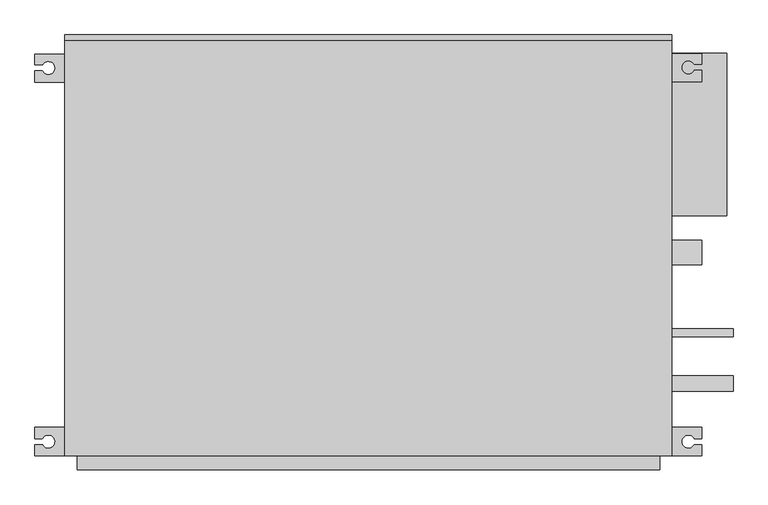
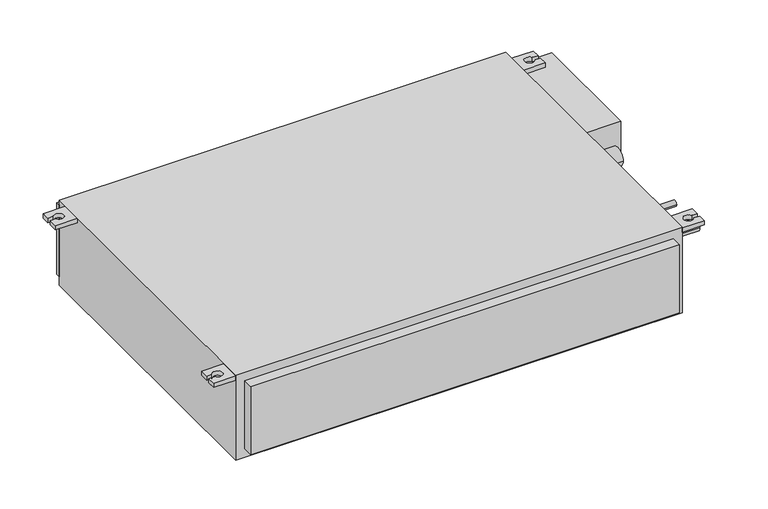
"""IFC4 building model written with IfcOpenShell, lengths in millimetres: proxy geometry, PEFY-P-NMSU-E_Low_Profile_Ducted : PEFY-P15NMSU-E."""

import ifcopenshell
import ifcopenshell.guid

model = None  # the IFC model being written
_history = None  # IfcOwnerHistory: only IFC2X3 demands one
_inside = {}  # id of a spatial element -> (the spatial element, [elements in it])
_under = {}  # id of a project, library or spatial element -> (it, [spatial elements below it])
_declared = {}  # id of a project -> (the project, [libraries it declares])
_typed = {}  # id of a type object -> (the type object, [elements of that type])
_made_of = {}  # id of a material, layer set ... -> (it, [elements and type objects made of it])


def new_model(schema):
    """Start an empty IFC model of exactly this schema.

    Asked for "IFC4X3", IfcOpenShell would pick the latest addendum, in which some entities
    have other attributes; the version numbers below select the first issue.
    IFC2X3 requires an IfcOwnerHistory on every rooted entity: one is made here for all.
    """
    global model, _history
    if schema == "IFC4X3":
        model = ifcopenshell.file(schema_version=(4, 3, 0, 0))
    else:
        model = ifcopenshell.file(schema=schema)
    _inside.clear()
    _under.clear()
    _declared.clear()
    _typed.clear()
    _made_of.clear()
    _history = None
    if model.schema == "IFC2X3":
        org = make("IfcOrganization", Name="unknown")
        user = make(
            "IfcPersonAndOrganization",
            ThePerson=make("IfcPerson", FamilyName="unknown"),
            TheOrganization=org,
        )
        app = make(
            "IfcApplication",
            ApplicationDeveloper=org,
            Version="unknown",
            ApplicationFullName="unknown",
            ApplicationIdentifier="unknown",
        )
        _history = make(
            "IfcOwnerHistory",
            OwningUser=user,
            OwningApplication=app,
            ChangeAction="ADDED",
            CreationDate=0,
        )
    return model


def make(cls, **values):
    """One entity of the class cls with the attributes given. An attribute that is None is left unset."""
    return model.create_entity(
        cls, **{name: value for name, value in values.items() if value is not None}
    )


def rooted(cls, **values):
    """An entity with a GlobalId (a new one), such as an element, a storey or a relation."""
    return make(cls, GlobalId=ifcopenshell.guid.new(), OwnerHistory=_history, **values)


def si_unit(unit_type, name, prefix=None):
    """IfcSIUnit, for example si_unit("LENGTHUNIT", "METRE", prefix="MILLI")."""
    return make("IfcSIUnit", UnitType=unit_type, Prefix=prefix, Name=name)


def assignment(units):
    """IfcUnitAssignment: the units of a project."""
    return None if units is None else make("IfcUnitAssignment", Units=units)


def point(xyz):
    """IfcCartesianPoint."""
    return None if xyz is None else make("IfcCartesianPoint", Coordinates=xyz)


def direction(xyz):
    """IfcDirection."""
    return None if xyz is None else make("IfcDirection", DirectionRatios=xyz)


def frame(location, z_axis=None, x_axis=None):
    """IfcAxis2Placement3D, a coordinate frame: its origin and axes. An axis left out is left unset."""
    return make(
        "IfcAxis2Placement3D",
        Location=point(location),
        Axis=direction(z_axis),
        RefDirection=direction(x_axis),
    )


def frame_2d(location, x_axis=None):
    """IfcAxis2Placement2D, a coordinate frame in the plane: its origin and x axis."""
    return make(
        "IfcAxis2Placement2D", Location=point(location), RefDirection=direction(x_axis)
    )


def origin():
    """The frame at (0, 0, 0) with its axes left unset."""
    return frame((0.0, 0.0, 0.0))


def origin_with_axes():
    """The frame at (0, 0, 0) with the z axis (0, 0, 1) and the x axis (1, 0, 0) written out."""
    return frame((0.0, 0.0, 0.0), z_axis=(0.0, 0.0, 1.0), x_axis=(1.0, 0.0, 0.0))


def place(relative_to, where):
    """IfcLocalPlacement: puts the frame where relative to a parent placement (None: the world)."""
    return make(
        "IfcLocalPlacement", PlacementRelTo=relative_to, RelativePlacement=where
    )


def context(
    kind, dimensions, precision=None, world=None, true_north=None, identifier=None
):
    """IfcGeometricRepresentationContext, for example the 3D "Model" context."""
    return make(
        "IfcGeometricRepresentationContext",
        ContextIdentifier=identifier,
        ContextType=kind,
        CoordinateSpaceDimension=dimensions,
        Precision=precision,
        WorldCoordinateSystem=world,
        TrueNorth=true_north,
    )


def project(units=None, contexts=None):
    """IfcProject with its units and contexts."""
    return rooted(
        "IfcProject",
        Name="project",
        RepresentationContexts=contexts,
        UnitsInContext=assignment(units),
    )


def spatial(cls, under=None, at=None, **own):
    """A site, building, storey or space (cls), placed at a placement, below another one or the project."""
    s = rooted(cls, ObjectPlacement=at, **own)
    if under is not None:
        _under.setdefault(under.id(), (under, []))[1].append(s)
    return s


def polyline(points):
    """IfcPolyline through the points."""
    return make("IfcPolyline", Points=[point(p) for p in points])


def circle_curve(where, radius):
    """IfcCircle in the frame where."""
    return make("IfcCircle", Position=where, Radius=radius)


def trimmed(basis, trim1, trim2, sense, master):
    """IfcTrimmedCurve: the piece of a basis curve between two trims."""
    return make(
        "IfcTrimmedCurve",
        BasisCurve=basis,
        Trim1=trim1,
        Trim2=trim2,
        SenseAgreement=sense,
        MasterRepresentation=master,
    )


def segment(curve, same_sense, transition):
    """IfcCompositeCurveSegment."""
    return make(
        "IfcCompositeCurveSegment",
        Transition=transition,
        SameSense=same_sense,
        ParentCurve=curve,
    )


def composite_curve(segments, self_intersect=None):
    """IfcCompositeCurve: segments joined end to end."""
    return make("IfcCompositeCurve", Segments=segments, SelfIntersect=self_intersect)


def outline(outer, holes=None, kind="AREA"):
    """IfcArbitraryClosedProfileDef: a profile drawn as a closed curve; with holes, ...WithVoids."""
    if holes is None:
        return make("IfcArbitraryClosedProfileDef", ProfileType=kind, OuterCurve=outer)
    return make(
        "IfcArbitraryProfileDefWithVoids",
        ProfileType=kind,
        OuterCurve=outer,
        InnerCurves=holes,
    )


def extrude(swept, where, along, depth):
    """IfcExtrudedAreaSolid: the profile swept, set in the frame where, extruded along a direction by depth."""
    return make(
        "IfcExtrudedAreaSolid",
        SweptArea=swept,
        Position=where,
        ExtrudedDirection=direction(along),
        Depth=depth,
    )


def shape(context_of_items, identifier, shape_type, items):
    """IfcShapeRepresentation: the items that make up one representation, for example the "Body"."""
    return make(
        "IfcShapeRepresentation",
        ContextOfItems=context_of_items,
        RepresentationIdentifier=identifier,
        RepresentationType=shape_type,
        Items=items,
    )


def source(mapping_origin, context_of_items, identifier, shape_type, items):
    """IfcRepresentationMap: a shape defined once, which mapped items show again and again."""
    return make(
        "IfcRepresentationMap",
        MappingOrigin=mapping_origin,
        MappedRepresentation=shape(context_of_items, identifier, shape_type, items),
    )


def transform(
    local_origin,
    x_axis=None,
    y_axis=None,
    z_axis=None,
    scale=None,
    scale2=None,
    scale3=None,
    uniform=True,
):
    """IfcCartesianTransformationOperator3D, or its non-uniform kind. x_axis, y_axis, z_axis: its Axis1, 2, 3."""
    if uniform:
        return make(
            "IfcCartesianTransformationOperator3D",
            Axis1=direction(x_axis),
            Axis2=direction(y_axis),
            LocalOrigin=point(local_origin),
            Scale=scale,
            Axis3=direction(z_axis),
        )
    return make(
        "IfcCartesianTransformationOperator3DnonUniform",
        Axis1=direction(x_axis),
        Axis2=direction(y_axis),
        LocalOrigin=point(local_origin),
        Scale=scale,
        Axis3=direction(z_axis),
        Scale2=scale2,
        Scale3=scale3,
    )


def mapped(mapping_source, mapping_target):
    """IfcMappedItem: shows the shape of a source again, moved by a transform."""
    return make(
        "IfcMappedItem", MappingSource=mapping_source, MappingTarget=mapping_target
    )


def made_of(thing, what):
    """Note that an element or type object is made of a material, layer set ...; save() writes the relation."""
    if what is not None:
        _made_of.setdefault(what.id(), (what, []))[1].append(thing)
    return thing


def element(
    cls,
    number,
    at=None,
    inside=None,
    cuts=None,
    type_object=None,
    material=None,
    context=None,
    identifier="Body",
    shape_type=None,
    held_by="IfcProductDefinitionShape",
    body=None,
    shapes=None,
    **own,
):
    """One element of the class cls, such as IfcWall. Its Tag is "e" and its number.

    at: its placement. inside: the storey or other place that contains it. cuts: it is an
    opening in that element (IfcRelVoidsElement). A single representation is given by context,
    identifier, shape_type and body (its items); several are given by shapes. held_by: the class
    of the entity that holds the representations. save() writes the other relations.
    """
    e = rooted(cls, Tag="e%d" % number, ObjectPlacement=at, **own)
    if body is not None:
        shapes = [shape(context, identifier, shape_type, body)]
    if shapes is not None:
        e.Representation = make(held_by, Representations=shapes)
    if inside is not None:
        _inside.setdefault(inside.id(), (inside, []))[1].append(e)
    if cuts is not None:
        rooted(
            "IfcRelVoidsElement", RelatingBuildingElement=cuts, RelatedOpeningElement=e
        )
    if type_object is not None:
        _typed.setdefault(type_object.id(), (type_object, []))[1].append(e)
    return made_of(e, material)


def aggregate(whole, parts):
    """IfcRelAggregates: a whole, such as a stair, and the parts it consists of."""
    return rooted("IfcRelAggregates", RelatingObject=whole, RelatedObjects=parts)


def save(model, path):
    """Write the relations noted so far, then the file.

    IfcRelAggregates (storeys below a building ...), IfcRelContainedInSpatialStructure (elements
    in a storey), IfcRelDefinesByType, IfcRelAssociatesMaterial and IfcRelDeclares: one each for
    every whole, place, type object, material and project.
    """
    for whole, parts in _under.values():
        aggregate(whole, parts)
    for where, things in _inside.values():
        rooted(
            "IfcRelContainedInSpatialStructure",
            RelatedElements=things,
            RelatingStructure=where,
        )
    for kind, things in _typed.values():
        rooted("IfcRelDefinesByType", RelatedObjects=things, RelatingType=kind)
    for what, things in _made_of.values():
        rooted("IfcRelAssociatesMaterial", RelatedObjects=things, RelatingMaterial=what)
    for by, libraries in _declared.values():
        rooted("IfcRelDeclares", RelatingContext=by, RelatedDefinitions=libraries)
    model.write(path)


def mechanical_equipment_be926906(model_context):
    return source(origin(), model_context, "Body", "SweptSolid", [
        extrude(outline(composite_curve([segment(polyline([(-544.3, 282.0), (-544.3, 300.9759165), (-532.1454311, 300.9759165)]), True, "CONTINUOUS"), segment(trimmed(circle_curve(frame_2d((-522.2863556, 305.4254582)), 10.8166442), [point((-532.1454311, 300.9759165))], [point((-531.8387803, 310.5))], True, "CARTESIAN"), True, "CONTINUOUS"), segment(polyline([(-531.8387803, 310.5), (-544.3, 310.5), (-544.3, 328.0), (-495.3, 328.0), (-495.3, 282.0), (-544.3, 282.0)]), True, "CONTINUOUS")], self_intersect=False)), frame((0.0, 0.0, 188.55), z_axis=(0.0, 0.0, 1.0), x_axis=(1.0, 0.0, 0.0)), (0.0, 0.0, 1.0), 10.0),
        extrude(outline(composite_curve([segment(polyline([(-544.3, -281.0), (-495.3, -281.0), (-495.3, -327.0), (-544.3, -327.0), (-544.3, -309.5), (-531.8387803, -309.5)]), True, "CONTINUOUS"), segment(trimmed(circle_curve(frame_2d((-522.2863556, -304.4254582)), 10.8166442), [point((-531.8387803, -309.5))], [point((-532.1454311, -299.9759165))], True, "CARTESIAN"), True, "CONTINUOUS"), segment(polyline([(-532.1454311, -299.9759165), (-544.3, -299.9759165), (-544.3, -281.0)]), True, "CONTINUOUS")], self_intersect=False)), frame((0.0, 0.0, 188.55), z_axis=(0.0, 0.0, 1.0), x_axis=(1.0, 0.0, 0.0)), (0.0, 0.0, 1.0), 10.0),
        extrude(outline(composite_curve([segment(polyline([(544.3, 282.9429009), (495.3, 282.9429009), (495.3, 328.9429009), (544.3, 328.9429009), (544.3, 311.4429009), (531.8387803, 311.4429009)]), True, "CONTINUOUS"), segment(trimmed(circle_curve(frame_2d((522.2863556, 306.3683591)), 10.8166442), [point((531.8387803, 311.4429009))], [point((532.1454311, 301.9188174))], True, "CARTESIAN"), True, "CONTINUOUS"), segment(polyline([(532.1454311, 301.9188174), (544.3, 301.9188174), (544.3, 282.9429009)]), True, "CONTINUOUS")], self_intersect=False)), frame((0.0, 0.0, 188.55), z_axis=(0.0, 0.0, 1.0), x_axis=(1.0, 0.0, 0.0)), (0.0, 0.0, 1.0), 10.0),
        extrude(outline(composite_curve([segment(polyline([(544.3, -281.0), (544.3, -299.9759165), (532.1454311, -299.9759165)]), True, "CONTINUOUS"), segment(trimmed(circle_curve(frame_2d((522.2863556, -304.4254582)), 10.8166442), [point((532.1454311, -299.9759165))], [point((531.8387803, -309.5))], True, "CARTESIAN"), True, "CONTINUOUS"), segment(polyline([(531.8387803, -309.5), (544.3, -309.5), (544.3, -327.0), (495.3, -327.0), (495.3, -281.0), (544.3, -281.0)]), True, "CONTINUOUS")], self_intersect=False)), frame((0.0, 0.0, 188.55), z_axis=(0.0, 0.0, 1.0), x_axis=(1.0, 0.0, 0.0)), (0.0, 0.0, 1.0), 10.0),
        extrude(outline(polyline([(495.3, 350.04375), (-495.3, 350.04375), (-495.3, 359.5477547), (495.3, 359.5477547), (495.3, 350.04375)])), frame((0.0, 0.0, 20.0), z_axis=(0.0, 0.0, 1.0), x_axis=(1.0, 0.0, 0.0)), (0.0, 0.0, 1.0), 168.55),
        extrude(outline(composite_curve([segment(trimmed(circle_curve(frame_2d((4.0570991, 59.8)), 20.0421875), [point((-15.9850884, 59.8))], [point((24.0992866, 59.8))], False, "CARTESIAN"), True, "CONTINUOUS"), segment(trimmed(circle_curve(frame_2d((4.0570991, 59.8)), 20.0421875), [point((24.0992866, 59.8))], [point((-15.9850884, 59.8))], False, "CARTESIAN"), True, "CONTINUOUS")], self_intersect=False)), frame((495.3, 0.0, 0.0), z_axis=(1.0, 0.0, 0.0), x_axis=(0.0, 1.0, 0.0)), (0.0, 0.0, 1.0), 26.9863556),
        extrude(outline(composite_curve([segment(trimmed(circle_curve(frame_2d((4.0570991, 149.6)), 20.0421875), [point((-15.9850884, 149.6))], [point((24.0992866, 149.6))], False, "CARTESIAN"), True, "CONTINUOUS"), segment(trimmed(circle_curve(frame_2d((4.0570991, 149.6)), 20.0421875), [point((24.0992866, 149.6))], [point((-15.9850884, 149.6))], False, "CARTESIAN"), True, "CONTINUOUS")], self_intersect=False)), frame((495.3, 0.0, 0.0), z_axis=(1.0, 0.0, 0.0), x_axis=(0.0, 1.0, 0.0)), (0.0, 0.0, 1.0), 49.0),
        extrude(outline(composite_curve([segment(trimmed(circle_curve(frame_2d((-126.5596979, 100.0)), 6.4492188), [point((-133.0089166, 100.0))], [point((-120.1104791, 100.0))], False, "CARTESIAN"), True, "CONTINUOUS"), segment(trimmed(circle_curve(frame_2d((-126.5596979, 100.0)), 6.4492188), [point((-120.1104791, 100.0))], [point((-133.0089166, 100.0))], False, "CARTESIAN"), True, "CONTINUOUS")], self_intersect=False)), frame((495.3, 0.0, 0.0), z_axis=(1.0, 0.0, 0.0), x_axis=(0.0, 1.0, 0.0)), (0.0, 0.0, 1.0), 100.0),
        extrude(outline(composite_curve([segment(trimmed(circle_curve(frame_2d((-209.7540575, 100.0)), 12.7), [point((-222.4540575, 100.0))], [point((-197.0540575, 100.0))], False, "CARTESIAN"), True, "CONTINUOUS"), segment(trimmed(circle_curve(frame_2d((-209.7540575, 100.0)), 12.7), [point((-197.0540575, 100.0))], [point((-222.4540575, 100.0))], False, "CARTESIAN"), True, "CONTINUOUS")], self_intersect=False)), frame((495.3, 0.0, 0.0), z_axis=(1.0, 0.0, 0.0), x_axis=(0.0, 1.0, 0.0)), (0.0, 0.0, 1.0), 100.0),
        extrude(outline(polyline([(585.3, 330.0), (585.3, 64.0570991), (495.3, 64.0570991), (495.3, 330.0), (585.3, 330.0)])), frame((0.0, 0.0, 20.0), z_axis=(0.0, 0.0, 1.0), x_axis=(1.0, 0.0, 0.0)), (0.0, 0.0, 1.0), 159.8),
        extrude(outline(polyline([(475.3, -350.04375), (-475.3, -350.04375), (-475.3, -327.0), (475.3, -327.0), (475.3, -350.04375)])), frame((0.0, 0.0, 19.9585938), z_axis=(0.0, 0.0, 1.0), x_axis=(1.0, 0.0, 0.0)), (0.0, 0.0, 1.0), 159.8414063),
        extrude(outline(polyline([(-495.3, -327.0), (-495.3, 350.04375), (495.3, 350.04375), (495.3, -327.0), (-495.3, -327.0)])), origin_with_axes(), (0.0, 0.0, 1.0), 200.0),
    ])


if __name__ == "__main__":
    model = new_model("IFC4")
    model_context = context("Model", 3, world=origin())
    ifc_project = project(units=[si_unit("LENGTHUNIT", "METRE", prefix="MILLI")], contexts=[model_context])
    site = spatial("IfcSite", under=ifc_project)
    building = spatial("IfcBuilding", under=site)
    placement = place(None, origin())
    mechanical_equipment_shape = mechanical_equipment_be926906(model_context)
    element("IfcBuildingElementProxy", 1, Name="PEFY-P-NMSU-E_Low_Profile_Ducted : PEFY-P15NMSU-E", ObjectType="PEFY-P-NMSU-E_Low_Profile_Ducted : PEFY-P15NMSU-E", at=placement, inside=building, context=model_context, shape_type="MappedRepresentation", body=[
        mapped(mechanical_equipment_shape, transform((0.0, 0.0, 0.0), x_axis=(1.0, 0.0, 0.0), y_axis=(0.0, 1.0, 0.0), z_axis=(0.0, 0.0, 1.0))),
    ])
    save(model, "model.ifc")

# Revit data of these elements
# Type "PEFY-P-NMSU-E_Low_Profile_Ducted : PEFY-P15NMSU-E"
#   Subcategory = "HVAC"
#   Standard Air Filter = "Polypropylene Honeycomb"
#   Specification URL = "http://www.mrslim.com/customerCare/resources.asp"
#   Sound Pressure Levels (dB(A)) = "28-30-33"
#   SmartBIM Object Created By = "Reed Construction Data"
#   Refirigerant Pipe diameter (Liquid) = "1/4\""
#   Refirigerant Pipe diameter (Gas) = "1/2\""
#   Power Source = "208/230, 1, 60"
#   Power Consumption Heating = "0.05 kW"
#   Power Consumption Cooling = "0.07 kW"
#   Unit Weight (LBS) = "54"
#   Model = "PEFY-P15NMSU-E"
#   Manufacturer URL = "http://www.mrslim.com/customerCare/resources.asp"
#   Manufacturer = "Mitsubishi Electric"
#   Installation URL = "http://www.mrslim.com/customerCare/resources.asp"
#   Fan Motor Type = "DC Motor"
#   Fan Motor Output = "0.096 kW"
#   MCA = "1.20/1.33"
#   MOCP = "15 A"
#   E.S.P (In. W.G.) = ".02-.20"
#   Drainpipe Dimension = "1-1/4"
#   Description = "Ceiling Concealed Ducted Low Profile"
#   Condensate Lift Mechanism = "21-11/16\" "
#   Coil Type = "Cross Fin"
#   Heating Capacity (BTU) = "17000"
#   Fan Type x Quantity = "Sirocco Fan x 2"
#   Current Heating = "0.45 A"
#   Current Cooling = "0.55 A"
#   Cooling Capacity (BTU) = "15000"
#   Fan capacity (CFM) = "282-335-388 "
#   Assembly Code = "D3050200"
#   95 CSI = "15760"
#   04 CSI = "23 82 19 "
#   Width = 990.6 mm
#   Voltage = 0 V
#   Unit Supply Airflow [instance default] = 0 CFM
#   Unit Return Airflow [instance default] = 0 CFM
#   SmartBIM Object Version = 3
#   Height = 200 mm
#   Drain Pipe Radius = 20.042 mm
#   Depth = 700.088 mm
#   Default Elevation = 1219.2 mm
#   C = 1088.6 mm
#   Brazing Connection Radius (Liquid) = 6.449 mm
#   Brazing Connection Radius (Gas) = 12.7 mm
#   Suspension Bolt Pitch = 1042.6 mm
#   Apparent Load = 0 VA
#   Air Outlet Width = 950.6 mm
#   Air Inlet Width = 990.6 mm
#   Air Outlet Height = 159.841 mm
#   Air Inlet Height = 169 mm
#   Number of Poles = 1
#   Load Classification = Other
#   External Finish = Galvanized Steel Sheet
#   Air Outlet Unit Material = Metal Grill
#   Air Inlet Unit Material = Grill
#   URL = ""
# Element 1 (IfcBuildingElementProxy, "PEFY-P-NMSU-E_Low_Profile_Ducted : PEFY-P15NMSU-E")
#   Unit Supply Airflow = 300 CFM
#   Unit Return Airflow = 400 CFM
#   Materials on its faces: "Galvanized Steel Sheet", "Grill", "Metal Grill"
# Materials
#   "Galvanized Steel Sheet": class "Metal", colour RGB 189 187 185, transparency 0
#   "Metal Grill": class "Metal", colour RGB 10 10 10, transparency 0
#   "Grill": class "Plastic", colour RGB 5 5 5, transparency 0
